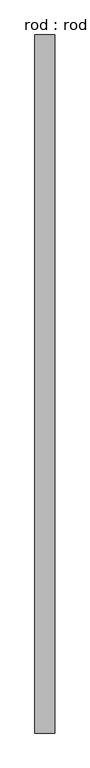
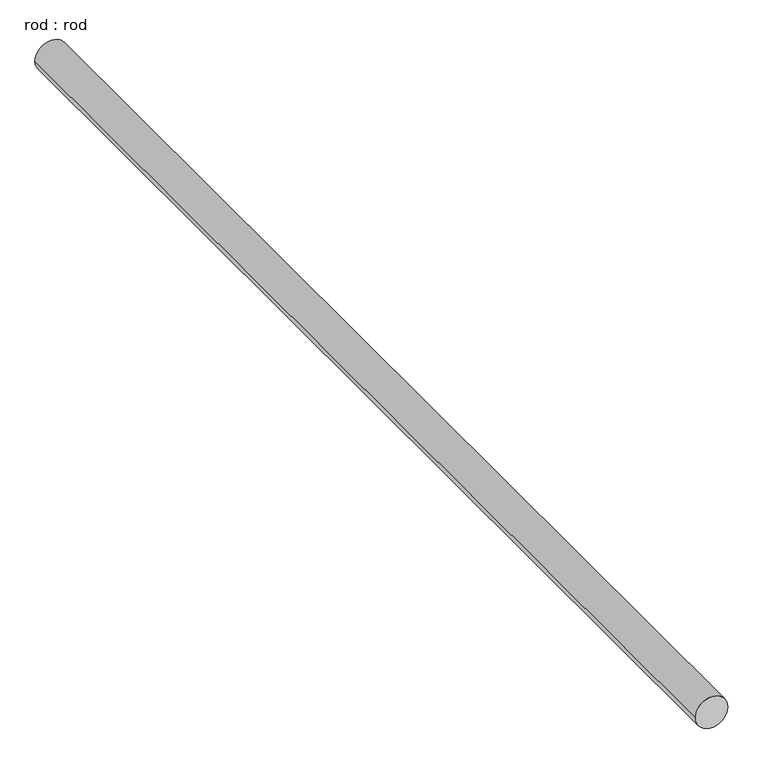
"""IFC4 building model written with IfcOpenShell, lengths in millimetres: proxy geometry, rod : rod."""

from ifc_helpers import new_model, si_unit, point, frame, frame_2d, origin, place, context, project, spatial, circle_curve, trimmed, segment, composite_curve, outline, extrude, source, transform, mapped, element, save


def rod_rod_aec1f85d(model_context):
    return source(origin(), model_context, "Body", "SweptSolid", [
        extrude(outline(composite_curve([segment(trimmed(circle_curve(frame_2d((0.0108462, 0.0)), 200.0), [point((0.0108462, 200.0))], [point((0.0108462, -200.0))], False, "CARTESIAN"), True, "CONTINUOUS"), segment(trimmed(circle_curve(frame_2d((0.0108462, 0.0)), 200.0), [point((0.0108462, -200.0))], [point((0.0108462, 200.0))], False, "CARTESIAN"), True, "CONTINUOUS")], self_intersect=False)), frame((0.0, -2910.8865226, 0.0), z_axis=(0.0, 1.0, 0.0), x_axis=(0.0, 0.0, 1.0)), (0.0, 0.0, 1.0), 14007.2302758),
    ])


if __name__ == "__main__":
    model = new_model("IFC4")
    model_context = context("Model", 3, world=origin())
    ifc_project = project(units=[si_unit("LENGTHUNIT", "METRE", prefix="MILLI")], contexts=[model_context])
    site = spatial("IfcSite", under=ifc_project)
    building = spatial("IfcBuilding", under=site)
    placement = place(None, origin())
    rod_rod_shape = rod_rod_aec1f85d(model_context)
    element("IfcBuildingElementProxy", 1, Name="rod : rod", ObjectType="rod : rod", at=placement, inside=building, context=model_context, shape_type="MappedRepresentation", body=[
        mapped(rod_rod_shape, transform((0.0, 0.0, 0.0), x_axis=(1.0, 0.0, 0.0), y_axis=(0.0, 1.0, 0.0), z_axis=(0.0, 0.0, 1.0))),
    ])
    save(model, "model.ifc")

# Revit data of these elements
# Type "rod : rod"
#   Default Elevation = 0
